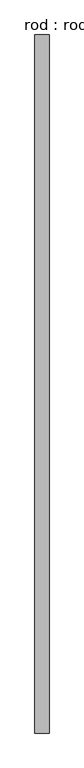
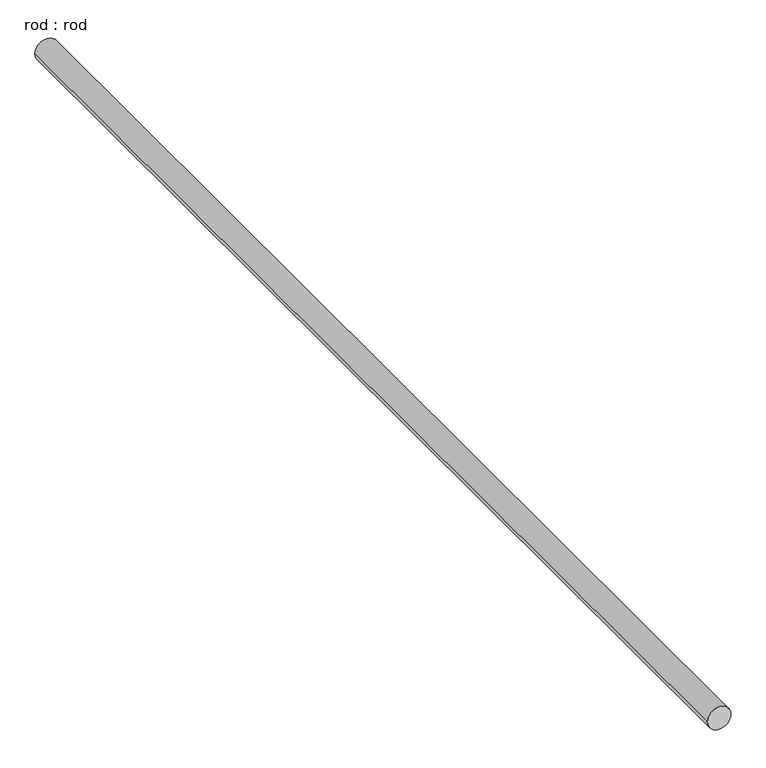
"""IFC4 building model written with IfcOpenShell, lengths in millimetres: proxy geometry, rod : rod."""

from ifc_helpers import new_model, si_unit, point, frame, frame_2d, origin, place, context, project, spatial, circle_curve, trimmed, segment, composite_curve, outline, extrude, source, transform, mapped, element, save


def rod_rod_81707754(model_context):
    return source(origin(), model_context, "Body", "SweptSolid", [
        extrude(outline(composite_curve([segment(trimmed(circle_curve(frame_2d((0.0108462, 0.0)), 200.0), [point((0.0108462, 200.0))], [point((0.0108462, -200.0))], False, "CARTESIAN"), True, "CONTINUOUS"), segment(trimmed(circle_curve(frame_2d((0.0108462, 0.0)), 200.0), [point((0.0108462, -200.0))], [point((0.0108462, 200.0))], False, "CARTESIAN"), True, "CONTINUOUS")], self_intersect=False)), frame((0.0, -5763.2749485, 0.0), z_axis=(0.0, 1.0, 0.0), x_axis=(0.0, 0.0, 1.0)), (0.0, 0.0, 1.0), 19712.0071276),
    ])


if __name__ == "__main__":
    model = new_model("IFC4")
    model_context = context("Model", 3, world=origin())
    ifc_project = project(units=[si_unit("LENGTHUNIT", "METRE", prefix="MILLI")], contexts=[model_context])
    site = spatial("IfcSite", under=ifc_project)
    building = spatial("IfcBuilding", under=site)
    placement = place(None, origin())
    rod_rod_shape = rod_rod_81707754(model_context)
    element("IfcBuildingElementProxy", 1, Name="rod : rod", ObjectType="rod : rod", at=placement, inside=building, context=model_context, shape_type="MappedRepresentation", body=[
        mapped(rod_rod_shape, transform((0.0, 0.0, 0.0), x_axis=(1.0, 0.0, 0.0), y_axis=(0.0, 1.0, 0.0), z_axis=(0.0, 0.0, 1.0))),
    ])
    save(model, "model.ifc")

# Revit data of these elements
# Type "rod : rod"
#   Default Elevation = 0
